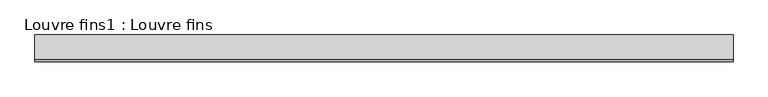
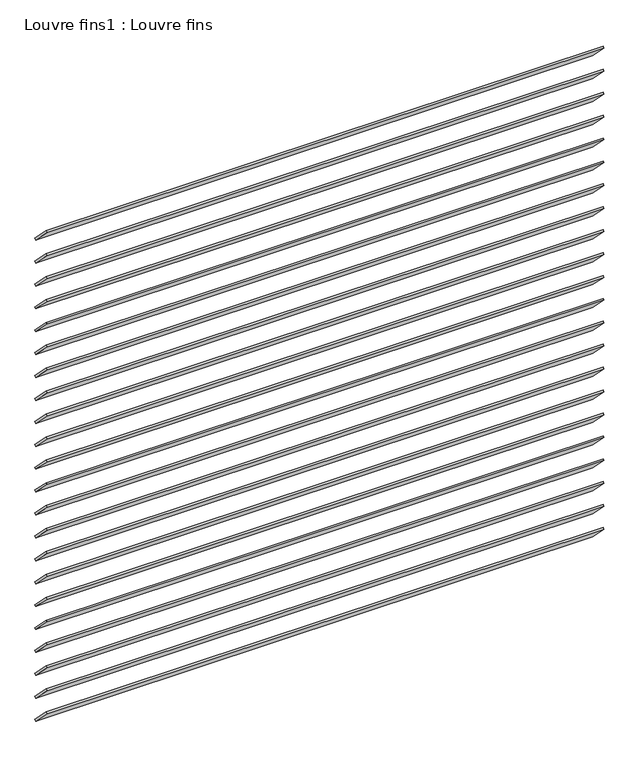
"""IFC4 building model written with IfcOpenShell, lengths in millimetres: proxy geometry, Louvre fins1 : Louvre fins."""

from ifc_helpers import new_model, si_unit, frame, origin, place, context, project, spatial, polyline, outline, extrude, source, transform, mapped, element, save


def louvre_fins1_louvre_fins_8b0860a4(model_context):
    return source(origin(), model_context, "Body", "SweptSolid", [
        extrude(outline(polyline([(0.0, -101.6), (0.0, 0.0), (2000.0, 0.0), (2000.0, -101.6), (0.0, -101.6)])), frame((3694.2883192, 9873.6979231, 37559.769849), z_axis=(0.0, 0.7071067811865476, 0.7071067811865476), x_axis=(1.0, 0.0, 0.0)), (0.0, 0.0, 1.0), 6.35),
        extrude(outline(polyline([(0.0, -101.6), (0.0, 0.0), (2000.0, 0.0), (2000.0, -101.6), (0.0, -101.6)])), frame((3694.2883192, 9873.6979231, 37646.769849), z_axis=(0.0, 0.7071067811865476, 0.7071067811865476), x_axis=(1.0, 0.0, 0.0)), (0.0, 0.0, 1.0), 6.35),
        extrude(outline(polyline([(0.0, -101.6), (0.0, 0.0), (2000.0, 0.0), (2000.0, -101.6), (0.0, -101.6)])), frame((3694.2883192, 9873.6979231, 37733.769849), z_axis=(0.0, 0.7071067811865476, 0.7071067811865476), x_axis=(1.0, 0.0, 0.0)), (0.0, 0.0, 1.0), 6.35),
        extrude(outline(polyline([(0.0, -101.6), (0.0, 0.0), (2000.0, 0.0), (2000.0, -101.6), (0.0, -101.6)])), frame((3694.2883192, 9873.6979231, 37820.769849), z_axis=(0.0, 0.7071067811865476, 0.7071067811865476), x_axis=(1.0, 0.0, 0.0)), (0.0, 0.0, 1.0), 6.35),
        extrude(outline(polyline([(0.0, -101.6), (0.0, 0.0), (2000.0, 0.0), (2000.0, -101.6), (0.0, -101.6)])), frame((3694.2883192, 9873.6979231, 37907.769849), z_axis=(0.0, 0.7071067811865476, 0.7071067811865476), x_axis=(1.0, 0.0, 0.0)), (0.0, 0.0, 1.0), 6.35),
        extrude(outline(polyline([(0.0, -101.6), (0.0, 0.0), (2000.0, 0.0), (2000.0, -101.6), (0.0, -101.6)])), frame((3694.2883192, 9873.6979231, 37994.769849), z_axis=(0.0, 0.7071067811865476, 0.7071067811865476), x_axis=(1.0, 0.0, 0.0)), (0.0, 0.0, 1.0), 6.35),
        extrude(outline(polyline([(0.0, -101.6), (0.0, 0.0), (2000.0, 0.0), (2000.0, -101.6), (0.0, -101.6)])), frame((3694.2883192, 9873.6979231, 38081.769849), z_axis=(0.0, 0.7071067811865476, 0.7071067811865476), x_axis=(1.0, 0.0, 0.0)), (0.0, 0.0, 1.0), 6.35),
        extrude(outline(polyline([(0.0, -101.6), (0.0, 0.0), (2000.0, 0.0), (2000.0, -101.6), (0.0, -101.6)])), frame((3694.2883192, 9873.6979231, 38168.769849), z_axis=(0.0, 0.7071067811865476, 0.7071067811865476), x_axis=(1.0, 0.0, 0.0)), (0.0, 0.0, 1.0), 6.35),
        extrude(outline(polyline([(0.0, -101.6), (0.0, 0.0), (2000.0, 0.0), (2000.0, -101.6), (0.0, -101.6)])), frame((3694.2883192, 9873.6979231, 38255.769849), z_axis=(0.0, 0.7071067811865476, 0.7071067811865476), x_axis=(1.0, 0.0, 0.0)), (0.0, 0.0, 1.0), 6.35),
        extrude(outline(polyline([(0.0, -101.6), (0.0, 0.0), (2000.0, 0.0), (2000.0, -101.6), (0.0, -101.6)])), frame((3694.2883192, 9873.6979231, 38342.769849), z_axis=(0.0, 0.7071067811865476, 0.7071067811865476), x_axis=(1.0, 0.0, 0.0)), (0.0, 0.0, 1.0), 6.35),
        extrude(outline(polyline([(0.0, -101.6), (0.0, 0.0), (2000.0, 0.0), (2000.0, -101.6), (0.0, -101.6)])), frame((3694.2883192, 9873.6979231, 38429.769849), z_axis=(0.0, 0.7071067811865476, 0.7071067811865476), x_axis=(1.0, 0.0, 0.0)), (0.0, 0.0, 1.0), 6.35),
        extrude(outline(polyline([(0.0, -101.6), (0.0, 0.0), (2000.0, 0.0), (2000.0, -101.6), (0.0, -101.6)])), frame((3694.2883192, 9873.6979231, 38516.769849), z_axis=(0.0, 0.7071067811865476, 0.7071067811865476), x_axis=(1.0, 0.0, 0.0)), (0.0, 0.0, 1.0), 6.35),
        extrude(outline(polyline([(0.0, -101.6), (0.0, 0.0), (2000.0, 0.0), (2000.0, -101.6), (0.0, -101.6)])), frame((3694.2883192, 9873.6979231, 38603.769849), z_axis=(0.0, 0.7071067811865369, 0.7071067811865582), x_axis=(1.0, 0.0, 0.0)), (0.0, 0.0, 1.0), 6.35),
        extrude(outline(polyline([(0.0, -101.6), (0.0, 0.0), (2000.0, 0.0), (2000.0, -101.6), (0.0, -101.6)])), frame((3694.2883192, 9873.6979231, 38690.769849), z_axis=(0.0, 0.7071067811865476, 0.7071067811865476), x_axis=(1.0, 0.0, 0.0)), (0.0, 0.0, 1.0), 6.35),
        extrude(outline(polyline([(0.0, -101.6), (0.0, 0.0), (2000.0, 0.0), (2000.0, -101.6), (0.0, -101.6)])), frame((3694.2883192, 9873.6979231, 38777.769849), z_axis=(0.0, 0.7071067811865476, 0.7071067811865476), x_axis=(1.0, 0.0, 0.0)), (0.0, 0.0, 1.0), 6.35),
        extrude(outline(polyline([(0.0, -101.6), (0.0, 0.0), (2000.0, 0.0), (2000.0, -101.6), (0.0, -101.6)])), frame((3694.2883192, 9873.6979231, 38864.769849), z_axis=(0.0, 0.7071067811865476, 0.7071067811865476), x_axis=(1.0, 0.0, 0.0)), (0.0, 0.0, 1.0), 6.35),
        extrude(outline(polyline([(0.0, -101.6), (0.0, 0.0), (2000.0, 0.0), (2000.0, -101.6), (0.0, -101.6)])), frame((3694.2883192, 9873.6979231, 38951.769849), z_axis=(0.0, 0.7071067811865689, 0.7071067811865263), x_axis=(1.0, 0.0, 0.0)), (0.0, 0.0, 1.0), 6.35),
        extrude(outline(polyline([(0.0, -101.6), (0.0, 0.0), (2000.0, 0.0), (2000.0, -101.6), (0.0, -101.6)])), frame((3694.2883192, 9873.6979231, 39038.769849), z_axis=(0.0, 0.7071067811865582, 0.7071067811865369), x_axis=(1.0, 0.0, 0.0)), (0.0, 0.0, 1.0), 6.35),
        extrude(outline(polyline([(0.0, -101.6), (0.0, 0.0), (2000.0, 0.0), (2000.0, -101.6), (0.0, -101.6)])), frame((3694.2883192, 9873.6979231, 39125.769849), z_axis=(0.0, 0.7071067811865263, 0.7071067811865689), x_axis=(1.0, 0.0, 0.0)), (0.0, 0.0, 1.0), 6.35),
        extrude(outline(polyline([(0.0, -101.6), (0.0, 0.0), (2000.0, 0.0), (2000.0, -101.6), (0.0, -101.6)])), frame((3694.2883192, 9873.6979231, 39212.769849), z_axis=(0.0, 0.7071067811865689, 0.7071067811865263), x_axis=(1.0, 0.0, 0.0)), (0.0, 0.0, 1.0), 6.35),
        extrude(outline(polyline([(0.0, -101.6), (0.0, 0.0), (2000.0, 0.0), (2000.0, -101.6), (0.0, -101.6)])), frame((3694.2883192, 9873.6979231, 39299.769849), z_axis=(0.0, 0.7071067811865263, 0.7071067811865689), x_axis=(1.0, 0.0, 0.0)), (0.0, 0.0, 1.0), 6.35),
        extrude(outline(polyline([(0.0, -101.6), (0.0, 0.0), (2000.0, 0.0), (2000.0, -101.6), (0.0, -101.6)])), frame((3694.2883192, 9873.6979231, 39386.769849), z_axis=(0.0, 0.7071067811865263, 0.7071067811865689), x_axis=(1.0, 0.0, 0.0)), (0.0, 0.0, 1.0), 6.35),
    ])


if __name__ == "__main__":
    model = new_model("IFC4")
    model_context = context("Model", 3, world=origin())
    ifc_project = project(units=[si_unit("LENGTHUNIT", "METRE", prefix="MILLI")], contexts=[model_context])
    site = spatial("IfcSite", under=ifc_project)
    building = spatial("IfcBuilding", under=site)
    placement = place(None, origin())
    louvre_fins1_louvre_fins_shape = louvre_fins1_louvre_fins_8b0860a4(model_context)
    element("IfcBuildingElementProxy", 1, Name="Louvre fins1 : Louvre fins", ObjectType="Louvre fins1 : Louvre fins", at=placement, inside=building, context=model_context, shape_type="MappedRepresentation", body=[
        mapped(louvre_fins1_louvre_fins_shape, transform((0.0, 0.0, 0.0), x_axis=(1.0, 0.0, 0.0), y_axis=(0.0, 1.0, 0.0), z_axis=(0.0, 0.0, 1.0))),
    ])
    save(model, "model.ifc")

# Revit data of these elements
# Type "Louvre fins1 : Louvre fins"
#   NameOverride = "Louvre fins"
# Element 1 (IfcBuildingElementProxy, "Louvre fins1 : Louvre fins")
#   Materials on its faces: "ALUMINIUM LOUVER - TBD"
# Materials
#   "ALUMINIUM LOUVER - TBD": class "Unassigned", colour RGB 92 107 122, transparency 0, Cost = 0
